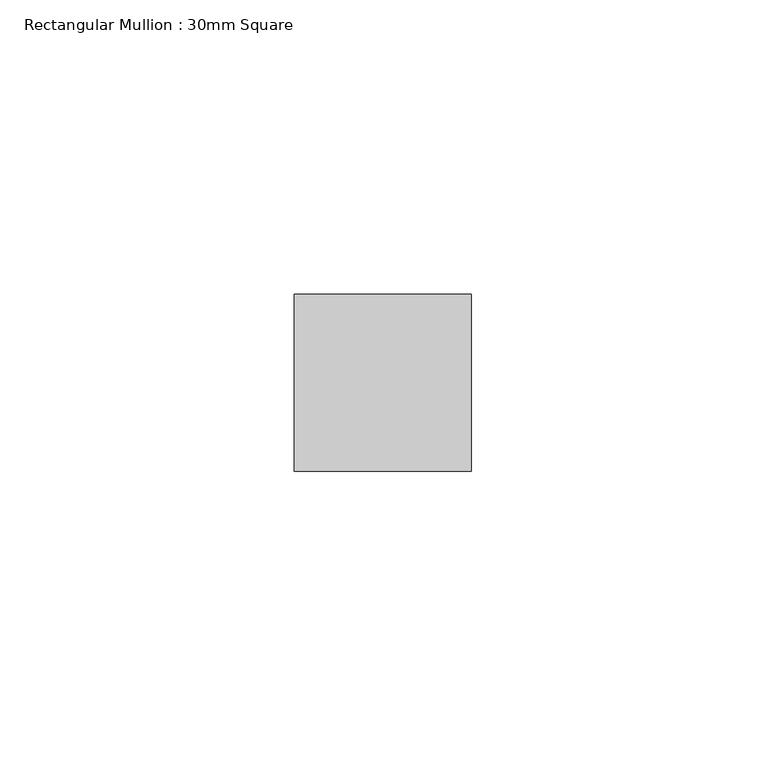
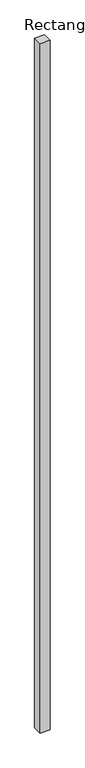
"""IFC4 building model written with IfcOpenShell, lengths in millimetres: member geometry, Rectangular Mullion : 30mm Square."""

from ifc_helpers import new_model, si_unit, frame, origin, place, context, project, spatial, polyline, outline, extrude, source, transform, mapped, element, save


def rectangular_mullion_30mm_square_3985f923(model_context):
    return source(origin(), model_context, "Body", "SweptSolid", [
        extrude(outline(polyline([(15.0, 15.0), (15.0, -15.0), (-15.0, -15.0), (-15.0, 15.0), (15.0, 15.0)])), frame((0.0, 0.0, -2270.73968), z_axis=(0.0, 0.0, 1.0), x_axis=(1.0, 0.0, 0.0)), (0.0, 0.0, 1.0), 2270.73968),
    ])


if __name__ == "__main__":
    model = new_model("IFC4")
    model_context = context("Model", 3, world=origin())
    ifc_project = project(units=[si_unit("LENGTHUNIT", "METRE", prefix="MILLI")], contexts=[model_context])
    site = spatial("IfcSite", under=ifc_project)
    building = spatial("IfcBuilding", under=site)
    placement = place(None, origin())
    rectangular_mullion_30mm_square_shape = rectangular_mullion_30mm_square_3985f923(model_context)
    element("IfcMember", 1, ObjectType="Rectangular Mullion : 30mm Square", at=placement, inside=building, context=model_context, shape_type="MappedRepresentation", body=[
        mapped(rectangular_mullion_30mm_square_shape, transform((0.0, 0.0, 0.0), x_axis=(1.0, 0.0, 0.0), y_axis=(0.0, 1.0, 0.0), z_axis=(0.0, 0.0, 1.0))),
    ])
    save(model, "model.ifc")

# Revit data of these elements
# Type "Rectangular Mullion : 30mm Square"
#   built-in parameter 1007304 = 0.0984252 (stored number, unit not read)
#   built-in parameter 1007301 = 0.0492126 (stored number, unit not read)
#   built-in parameter 1007300 = 0.0492126 (stored number, unit not read)
# Element 1 (IfcMember, "Rectangular Mullion : 30mm Square")
#   Materials on its faces: "Aluminum"
# Materials
#   "Aluminum": class "Metal", colour RGB 244 244 244, transparency 0, Description = "Aluminum 6061", Cost = 0
